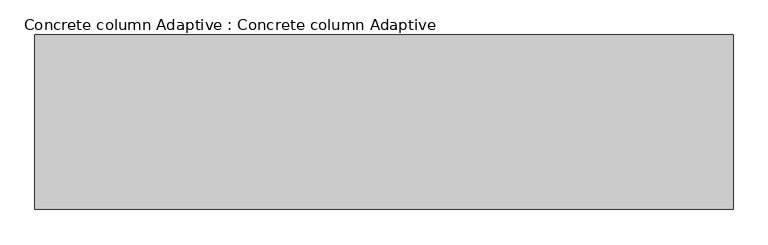
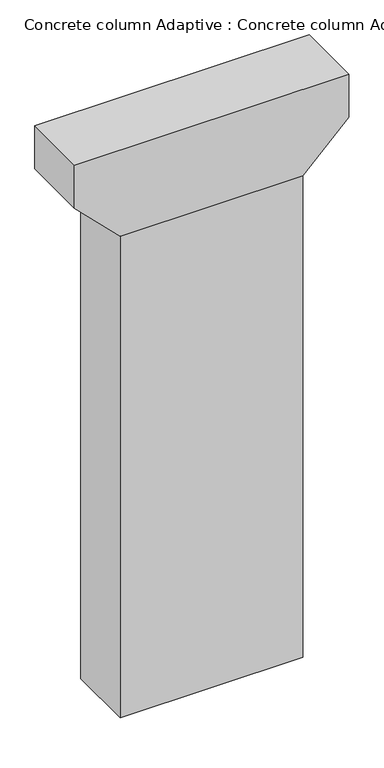
"""IFC4 building model written with IfcOpenShell, lengths in millimetres: proxy geometry, Concrete column Adaptive : Concrete column Adaptive."""

from ifc_helpers import new_model, si_unit, frame, origin, origin_with_axes, place, context, project, spatial, polyline, outline, extrude, source, transform, mapped, element, save


def concrete_column_adaptive_concrete_column_adaptive_6c7a738b(model_context):
    return source(origin(), model_context, "Body", "SweptSolid", [
        extrude(outline(polyline([(26284.0, 6000.0), (26284.0, -6000.0), (24284.0, -6000.0), (22284.0, -4000.0), (22284.0, 4000.0), (24284.0, 6000.0), (26284.0, 6000.0)])), frame((0.0, -1500.0, 0.0), z_axis=(0.0, 1.0, 0.0), x_axis=(0.0, 0.0, 1.0)), (0.0, 0.0, 1.0), 3000.0),
        extrude(outline(polyline([(-4000.0, -1500.0), (-4000.0, 1500.0), (4000.0, 1500.0), (4000.0, -1500.0), (-4000.0, -1500.0)])), origin_with_axes(), (0.0, 0.0, 1.0), 22284.0),
    ])


if __name__ == "__main__":
    model = new_model("IFC4")
    model_context = context("Model", 3, world=origin())
    ifc_project = project(units=[si_unit("LENGTHUNIT", "METRE", prefix="MILLI")], contexts=[model_context])
    site = spatial("IfcSite", under=ifc_project)
    building = spatial("IfcBuilding", under=site)
    placement = place(None, origin())
    concrete_column_adaptive_concrete_column_adaptive_shape = concrete_column_adaptive_concrete_column_adaptive_6c7a738b(model_context)
    element("IfcBuildingElementProxy", 1, Name="Concrete column Adaptive : Concrete column Adaptive", ObjectType="Concrete column Adaptive : Concrete column Adaptive", at=placement, inside=building, context=model_context, shape_type="MappedRepresentation", body=[
        mapped(concrete_column_adaptive_concrete_column_adaptive_shape, transform((0.0, 0.0, 0.0), x_axis=(1.0, 0.0, 0.0), y_axis=(0.0, 1.0, 0.0), z_axis=(0.0, 0.0, 1.0))),
    ])
    save(model, "model.ifc")

# Revit data of these elements
# Type "Concrete column Adaptive : Concrete column Adaptive"
#   Height [instance default] = 30000 mm
#   Default Elevation = 0
# Element 1 (IfcBuildingElementProxy, "Concrete column Adaptive : Concrete column Adaptive")
#   Height = 22284 mm
